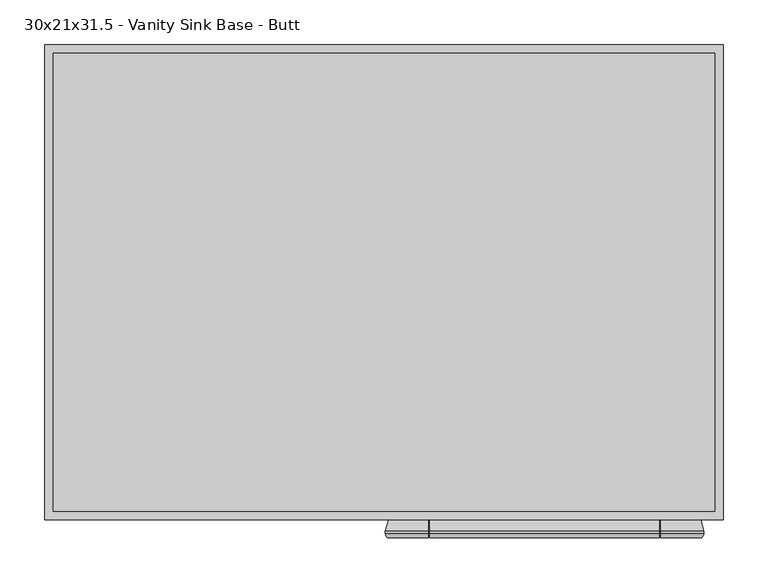
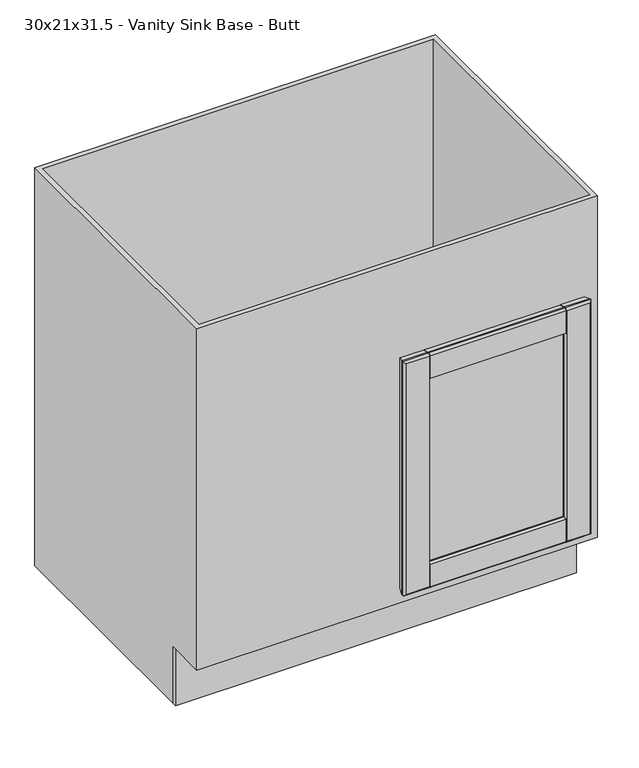
"""IFC4 building model written with IfcOpenShell, lengths in millimetres: furniture geometry, Cabinet-Base-Merillat-Double_Door-Marlin : 30x21x31.5 - Vanity Sink Base - Butt."""

from ifc_helpers import new_model, si_unit, frame, origin, origin_with_axes, place, context, project, spatial, polyline, circle_curve, ellipse_curve, outline, extrude, faceted_brep, source, transform, mapped, element, save
from ifc_brep_helpers import plane_surface, cylinder_surface, advanced_brep


def furniture_30x21x31_5_vanity_sink_base_butt_bc92859f(model_context):
    return source(origin(), model_context, "Body", "SolidModel", [
        advanced_brep(
        [(377.5127049, -625.4496, 609.6), (374.4162124, -629.92, 606.5035075), (374.4162124, -629.92, 142.7964925), (377.5127049, -625.4496, 139.7), (377.5127049, -622.681, 139.7), (377.5127049, -622.681, 609.6), (374.0075049, -609.6, 143.2052), (374.0075049, -609.6, 606.0948), (329.3115422, -609.6, 561.3988372), (329.3115422, -609.6, 187.9011628), (328.9414105, -610.39375, 188.2712945), (326.8602514, -614.85681, 190.3524535), (326.8602514, -614.85681, 558.9475465), (328.9414105, -610.39375, 561.0287055), (328.2600209, -617.0969093, 188.952684), (328.2600209, -617.0969093, 560.347316), (342.5877049, -617.347, 174.625), (342.5877049, -617.347, 574.675), (342.5877049, -622.173, 174.625), (342.5877049, -622.173, 574.675), (328.2600209, -622.4230907, 188.952684), (328.2600209, -622.4230907, 560.347316), (326.8602514, -624.66319, 190.3524535), (326.8602514, -624.66319, 558.9475465), (328.9414105, -629.12625, 188.2712945), (329.3086747, -629.9138508, 187.9040302), (329.3115422, -629.92, 561.3988372), (328.9414105, -629.12625, 561.0287055), (329.3086747, -629.92, 142.7964925), (329.3086747, -625.4496, 139.7), (23.4216974, -629.92, 142.7964925), (20.3252049, -625.4496, 139.7), (68.4894236, -625.4496, 139.7), (68.4894236, -629.92, 142.7964925), (327.7211747, -625.4496, 139.7), (327.7211747, -629.92, 142.7964925), (70.0769236, -629.92, 142.7964925), (70.0769236, -625.4496, 139.7), (329.3086747, -622.681, 139.7), (20.3252049, -622.681, 139.7), (68.4894236, -622.681, 139.7), (327.7211747, -622.681, 139.7), (70.0769236, -622.681, 139.7), (329.3086747, -609.6, 143.2052), (23.8304049, -609.6, 143.2052), (68.4894236, -609.6, 143.2052), (327.7211747, -609.6, 143.2052), (70.0769236, -609.6, 143.2052), (70.9776584, -614.85681, 190.3524535), (327.7211747, -610.39375, 188.2712945), (327.7211747, -609.6, 187.9011628), (70.0769236, -609.6, 187.9011628), (70.0769236, -610.39375, 188.2712945), (68.8964994, -610.39375, 188.2712945), (69.577889, -617.0969093, 188.952684), (55.2502049, -617.347, 174.625), (55.2502049, -622.173, 174.625), (69.577889, -622.4230907, 188.952684), (70.9776584, -624.66319, 190.3524535), (68.8964994, -629.12625, 188.2712945), (70.0769236, -629.12625, 188.2712945), (70.0769236, -629.92, 187.9011628), (327.7211747, -629.92, 187.9011628), (327.7211747, -629.12625, 188.2712945), (23.4216974, -629.92, 606.5035075), (20.3252049, -625.4496, 609.6), (20.3252049, -622.681, 609.6), (23.8304049, -609.6, 606.0948), (68.5263677, -609.6, 187.9011628), (68.5263677, -609.6, 561.3988372), (68.8964994, -610.39375, 561.0287055), (70.9776584, -614.85681, 558.9475465), (69.577889, -617.0969093, 560.347316), (55.2502049, -617.347, 574.675), (55.2502049, -622.173, 574.675), (69.577889, -622.4230907, 560.347316), (70.9776584, -624.66319, 558.9475465), (68.8964994, -629.12625, 561.0287055), (68.5263677, -629.92, 561.3988372), (68.5263677, -629.92, 187.9011628), (68.4894236, -629.92, 606.5035075), (68.4894236, -625.4496, 609.6), (329.3086747, -625.4496, 609.6), (329.3086747, -629.92, 606.5035075), (70.0769236, -625.4496, 609.6), (70.0769236, -629.92, 606.5035075), (327.7211747, -629.92, 606.5035075), (327.7211747, -625.4496, 609.6), (68.4894236, -622.681, 609.6), (329.3086747, -622.681, 609.6), (70.0769236, -622.681, 609.6), (327.7211747, -622.681, 609.6), (68.4894236, -609.6, 606.0948), (329.3086747, -609.6, 606.0948), (70.0769236, -609.6, 606.0948), (327.7211747, -609.6, 606.0948), (70.0769236, -609.6, 561.3988372), (327.7211747, -609.6, 561.3988372), (70.0769236, -610.39375, 561.0287055), (327.7211747, -610.39375, 561.0287055), (327.7211747, -629.12625, 561.0287055), (327.7211747, -629.92, 561.3988372), (70.0769236, -629.92, 561.3988372), (70.0769236, -629.12625, 561.0287055), (70.0769236, -610.39375, 605.4857412), (70.0769236, -622.7855037, 608.80625), (70.0769236, -625.4496, 608.80625), (70.0769236, -629.12625, 606.3526052), (68.4894236, -629.12625, 561.0287055), (68.4894236, -629.12625, 606.3526052), (68.4894236, -625.4496, 608.80625), (68.4894236, -622.7855037, 608.80625), (68.4894236, -610.39375, 605.4857412), (68.4894236, -610.39375, 561.0287055), (329.3086747, -610.39375, 561.0287055), (329.3086747, -610.39375, 605.4857412), (329.3086747, -622.7855037, 608.80625), (329.3086747, -625.4496, 608.80625), (329.3086747, -629.12625, 606.3526052), (329.3086747, -629.12625, 561.0287055), (327.7211747, -629.12625, 606.3526052), (327.7211747, -625.4496, 608.80625), (327.7211747, -622.7855037, 608.80625), (327.7211747, -610.39375, 605.4857412), (329.3086747, -629.12625, 188.2712945), (329.3086747, -629.12625, 142.9473948), (329.3086747, -625.4496, 140.49375), (329.3086747, -622.7855037, 140.49375), (329.3086747, -610.39375, 143.8142588), (329.3086747, -610.39375, 188.2712945), (327.7211747, -610.39375, 143.8142588), (327.7211747, -622.7855037, 140.49375), (327.7211747, -625.4496, 140.49375), (327.7211747, -629.12625, 142.9473948), (70.0769236, -629.12625, 142.9473948), (70.0769236, -625.4496, 140.49375), (70.0769236, -622.7855037, 140.49375), (70.0769236, -610.39375, 143.8142588), (68.4894236, -629.12625, 188.2712945), (68.4894236, -610.39375, 188.2712945), (68.4894236, -610.39375, 143.8142588), (68.4894236, -622.7855037, 140.49375), (68.4894236, -625.4496, 140.49375), (68.4894236, -629.12625, 142.9473948)],
        [
            (0, 1, ellipse_curve(frame((372.7375049, -625.4496, 604.8248), z_axis=(0.7071067811865475, 0.0, -0.7071067811865475), x_axis=(0.7071067811865474, 0.0, 0.7071067811865476)), 6.7531526, 4.7752)),
            (1, 2),
            (2, 3, ellipse_curve(frame((372.7375049, -625.4496, 144.4752), z_axis=(0.7071067811865475, 0.0, 0.7071067811865475), x_axis=(-0.7071067811865474, 0.0, 0.7071067811865476)), 6.7531526, 4.7752)),
            (3, 0),
            (3, 4),
            (4, 5),
            (5, 0),
            (4, 6),
            (6, 7),
            (7, 5),
            (8, 9),
            (9, 10),
            (10, 11),
            (11, 12),
            (12, 13),
            (13, 8),
            (11, 14, ellipse_curve(frame((328.2875049, -615.5223492, 188.9252), z_axis=(0.7071067811865475, 0.0, 0.7071067811865475), x_axis=(-0.7071067811865474, 0.0, 0.7071067811865476)), 2.2271035, 1.5748)),
            (14, 15),
            (15, 12, ellipse_curve(frame((328.2875049, -615.5223492, 560.3748), z_axis=(0.7071067811865475, 0.0, -0.7071067811865475), x_axis=(0.7071067811865474, 0.0, 0.7071067811865476)), 2.2271035, 1.5748)),
            (14, 16),
            (16, 17),
            (17, 15),
            (16, 18),
            (18, 19),
            (19, 17),
            (18, 20),
            (20, 21),
            (21, 19),
            (20, 22, ellipse_curve(frame((328.2875049, -623.9976508, 188.9252), z_axis=(0.7071067811865475, 0.0, 0.7071067811865475), x_axis=(-0.7071067811865474, 0.0, 0.7071067811865476)), 2.2271035, 1.5748)),
            (22, 23),
            (23, 21, ellipse_curve(frame((328.2875049, -623.9976508, 560.3748), z_axis=(0.7071067811865475, 0.0, -0.7071067811865475), x_axis=(0.7071067811865474, 0.0, 0.7071067811865476)), 2.2271035, 1.5748)),
            (22, 24),
            (24, 25),
            (25, 26),
            (26, 27),
            (27, 23),
            (2, 28),
            (28, 29, circle_curve(frame((329.3086747, -625.4496, 144.4752), z_axis=(1.0, 0.0, 0.0), x_axis=(0.0, 1.0, 0.0)), 4.7752)),
            (29, 3),
            (30, 31, ellipse_curve(frame((25.1004049, -625.4496, 144.4752), z_axis=(0.7071067811865475, 0.0, -0.7071067811865475), x_axis=(0.7071067811865476, 0.0, 0.7071067811865474)), 6.7531526, 4.7752)),
            (31, 32),
            (32, 33, circle_curve(frame((68.4894236, -625.4496, 144.4752), z_axis=(-1.0, 0.0, 0.0), x_axis=(0.0, 1.0, 0.0)), 4.7752)),
            (33, 30),
            (34, 35, circle_curve(frame((327.7211747, -625.4496, 144.4752), z_axis=(-1.0, 0.0, 0.0), x_axis=(0.0, 1.0, 0.0)), 4.7752)),
            (35, 36),
            (36, 37, circle_curve(frame((70.0769236, -625.4496, 144.4752), z_axis=(1.0, 0.0, 0.0), x_axis=(0.0, 1.0, 0.0)), 4.7752)),
            (37, 34),
            (29, 38),
            (38, 4),
            (31, 39),
            (39, 40),
            (40, 32),
            (41, 34),
            (37, 42),
            (42, 41),
            (38, 43),
            (43, 6),
            (39, 44),
            (44, 45),
            (45, 40),
            (46, 41),
            (42, 47),
            (47, 46),
            (48, 11),
            (10, 49),
            (49, 50),
            (50, 51),
            (51, 52),
            (52, 53),
            (53, 48),
            (48, 54, ellipse_curve(frame((69.5504049, -615.5223492, 188.9252), z_axis=(0.7071067811865475, 0.0, -0.7071067811865475), x_axis=(0.7071067811865476, 0.0, 0.7071067811865474)), 2.2271035, 1.5748)),
            (54, 14),
            (54, 55),
            (55, 16),
            (55, 56),
            (56, 18),
            (56, 57),
            (57, 20),
            (57, 58, ellipse_curve(frame((69.5504049, -623.9976508, 188.9252), z_axis=(0.7071067811865475, 0.0, -0.7071067811865475), x_axis=(0.7071067811865476, 0.0, 0.7071067811865474)), 2.2271035, 1.5748)),
            (58, 22),
            (58, 59),
            (59, 60),
            (60, 61),
            (61, 62),
            (62, 63),
            (63, 24),
            (30, 64),
            (64, 65, ellipse_curve(frame((25.1004049, -625.4496, 604.8248), z_axis=(-0.7071067811865475, 0.0, -0.7071067811865475), x_axis=(0.7071067811865474, 0.0, -0.7071067811865476)), 6.7531526, 4.7752)),
            (65, 31),
            (65, 66),
            (66, 39),
            (66, 67),
            (67, 44),
            (68, 69),
            (69, 70),
            (70, 71),
            (71, 48),
            (53, 68),
            (71, 72, ellipse_curve(frame((69.5504049, -615.5223492, 560.3748), z_axis=(-0.7071067811865475, 0.0, -0.7071067811865475), x_axis=(0.7071067811865474, 0.0, -0.7071067811865476)), 2.2271035, 1.5748)),
            (72, 54),
            (72, 73),
            (73, 55),
            (73, 74),
            (74, 56),
            (74, 75),
            (75, 57),
            (75, 76, ellipse_curve(frame((69.5504049, -623.9976508, 560.3748), z_axis=(-0.7071067811865475, 0.0, -0.7071067811865475), x_axis=(0.7071067811865474, 0.0, -0.7071067811865476)), 2.2271035, 1.5748)),
            (76, 58),
            (76, 77),
            (77, 78),
            (78, 79),
            (79, 59),
            (64, 80),
            (80, 81, circle_curve(frame((68.4894236, -625.4496, 604.8248), z_axis=(-1.0, 0.0, 0.0), x_axis=(0.0, 1.0, 0.0)), 4.7752)),
            (81, 65),
            (0, 82),
            (82, 83, circle_curve(frame((329.3086747, -625.4496, 604.8248), z_axis=(1.0, 0.0, 0.0), x_axis=(0.0, 1.0, 0.0)), 4.7752)),
            (83, 1),
            (84, 85, circle_curve(frame((70.0769236, -625.4496, 604.8248), z_axis=(1.0, 0.0, 0.0), x_axis=(0.0, 1.0, 0.0)), 4.7752)),
            (85, 86),
            (86, 87, circle_curve(frame((327.7211747, -625.4496, 604.8248), z_axis=(-1.0, 0.0, 0.0), x_axis=(0.0, 1.0, 0.0)), 4.7752)),
            (87, 84),
            (81, 88),
            (88, 66),
            (5, 89),
            (89, 82),
            (90, 84),
            (87, 91),
            (91, 90),
            (88, 92),
            (92, 67),
            (7, 93),
            (93, 89),
            (94, 90),
            (91, 95),
            (95, 94),
            (43, 9),
            (8, 93),
            (92, 69),
            (68, 45),
            (96, 94),
            (95, 97),
            (97, 96),
            (50, 46),
            (47, 51),
            (12, 71),
            (70, 98),
            (98, 96),
            (97, 99),
            (99, 13),
            (15, 72),
            (17, 73),
            (19, 74),
            (21, 75),
            (23, 76),
            (27, 100),
            (100, 101),
            (101, 102),
            (102, 103),
            (103, 77),
            (83, 26),
            (25, 28),
            (33, 79),
            (78, 80),
            (85, 102),
            (101, 86),
            (35, 62),
            (61, 36),
            (98, 104),
            (104, 105),
            (105, 106),
            (106, 107, circle_curve(frame((70.0769236, -625.4496, 604.8248), z_axis=(1.0, 0.0, 0.0), x_axis=(0.0, 0.0, 1.0)), 3.98145)),
            (107, 103),
            (78, 108),
            (108, 109),
            (109, 110, circle_curve(frame((68.4894236, -625.4496, 604.8248), z_axis=(-1.0, 0.0, 0.0), x_axis=(0.0, 0.0, 1.0)), 3.98145)),
            (110, 111),
            (111, 112),
            (112, 113),
            (113, 69),
            (77, 108),
            (107, 109),
            (106, 110),
            (105, 111),
            (104, 112),
            (70, 113),
            (8, 114),
            (114, 115),
            (115, 116),
            (116, 117),
            (117, 118, circle_curve(frame((329.3086747, -625.4496, 604.8248), z_axis=(1.0, 0.0, 0.0), x_axis=(0.0, 0.0, 1.0)), 3.98145)),
            (118, 119),
            (119, 26),
            (100, 120),
            (120, 121, circle_curve(frame((327.7211747, -625.4496, 604.8248), z_axis=(-1.0, 0.0, 0.0), x_axis=(0.0, 0.0, 1.0)), 3.98145)),
            (121, 122),
            (122, 123),
            (123, 99),
            (119, 27),
            (118, 120),
            (117, 121),
            (116, 122),
            (115, 123),
            (114, 13),
            (25, 124),
            (124, 125),
            (125, 126, circle_curve(frame((329.3086747, -625.4496, 144.4752), z_axis=(1.0, 0.0, 0.0), x_axis=(0.0, 0.0, 1.0)), 3.98145)),
            (126, 127),
            (127, 128),
            (128, 129),
            (129, 9),
            (49, 130),
            (130, 131),
            (131, 132),
            (132, 133, circle_curve(frame((327.7211747, -625.4496, 144.4752), z_axis=(-1.0, 0.0, 0.0), x_axis=(0.0, 0.0, 1.0)), 3.98145)),
            (133, 63),
            (129, 10),
            (128, 130),
            (127, 131),
            (126, 132),
            (125, 133),
            (124, 24),
            (60, 134),
            (134, 135, circle_curve(frame((70.0769236, -625.4496, 144.4752), z_axis=(1.0, 0.0, 0.0), x_axis=(0.0, 0.0, 1.0)), 3.98145)),
            (135, 136),
            (136, 137),
            (137, 52),
            (138, 79),
            (68, 139),
            (139, 140),
            (140, 141),
            (141, 142),
            (142, 143, circle_curve(frame((68.4894236, -625.4496, 144.4752), z_axis=(-1.0, 0.0, 0.0), x_axis=(0.0, 0.0, 1.0)), 3.98145)),
            (143, 138),
            (138, 59),
            (53, 139),
            (137, 140),
            (136, 141),
            (135, 142),
            (134, 143),
        ],
        [
            cylinder_surface(frame((372.7375049, -625.4496, 609.6), z_axis=(0.0, 0.0, 1.0), x_axis=(0.0, 1.0, 0.0)), 4.7752),
            plane_surface(frame((377.5127049, -625.4496, 609.6), z_axis=(1.0, 0.0, 0.0), x_axis=(0.0, 0.0, -1.0))),
            plane_surface(frame((377.5127049, -622.681, 609.6), z_axis=(0.9659229350723619, 0.25882983502910506, 0.0), x_axis=(0.0, 0.0, -1.0))),
            plane_surface(frame((329.3115422, -609.6, 561.3988372), z_axis=(-0.9063077870366099, 0.4226182617407856, 0.0), x_axis=(0.0, 0.0, -1.0))),
            cylinder_surface(frame((328.2875049, -615.5223492, 609.6), z_axis=(0.0, 0.0, 1.0000000000000002), x_axis=(-0.01745240643729364, -0.9998476951563912, 0.0)), 1.5748),
            plane_surface(frame((328.2600209, -617.0969093, 560.347316), z_axis=(-0.017452406437322144, -0.9998476951563906, 0.0), x_axis=(0.0, 0.0, -1.0))),
            plane_surface(frame((342.5877049, -617.347, 574.675), z_axis=(-1.0, 0.0, 0.0), x_axis=(0.0, 0.0, -1.0))),
            plane_surface(frame((342.5877049, -622.173, 574.675), z_axis=(-0.01745240643727848, 0.9998476951563914, 0.0), x_axis=(0.0, 0.0, -1.0))),
            cylinder_surface(frame((328.2875049, -623.9976508, 609.6), z_axis=(0.0, 0.0, 1.0000000000000002), x_axis=(-0.9063077870367326, -0.42261826174052236, 0.0)), 1.5748),
            plane_surface(frame((326.8602514, -624.66319, 558.9475465), z_axis=(-0.9063077870366333, -0.4226182617407352, 0.0), x_axis=(0.0, 0.0, -1.0))),
            cylinder_surface(frame((377.5127049, -625.4496, 144.4752), z_axis=(1.0, 0.0, 0.0), x_axis=(0.0, 1.0, 0.0)), 4.7752),
            plane_surface(frame((377.5127049, -625.4496, 139.7), z_axis=(0.0, 0.0, -1.0), x_axis=(-1.0, 0.0, 0.0))),
            plane_surface(frame((377.5127049, -622.681, 139.7), z_axis=(0.0, 0.25882983502910506, -0.9659229350723619), x_axis=(-1.0, 0.0, 0.0))),
            plane_surface(frame((329.3115422, -609.6, 187.9011628), z_axis=(0.0, 0.4226182617407856, 0.9063077870366099), x_axis=(-1.0, 0.0, 0.0))),
            cylinder_surface(frame((377.5127049, -615.5223492, 188.9252), z_axis=(1.0000000000000002, 0.0, 0.0), x_axis=(0.0, -0.9998476951563912, 0.01745240643729364)), 1.5748),
            plane_surface(frame((328.2600209, -617.0969093, 188.952684), z_axis=(0.0, -0.9998476951563906, 0.017452406437322144), x_axis=(-1.0, 0.0, 0.0))),
            plane_surface(frame((342.5877049, -617.347, 174.625), z_axis=(0.0, 0.0, 1.0), x_axis=(-1.0, 0.0, 0.0))),
            plane_surface(frame((342.5877049, -622.173, 174.625), z_axis=(0.0, 0.9998476951563914, 0.01745240643727848), x_axis=(-1.0, 0.0, 0.0))),
            cylinder_surface(frame((377.5127049, -623.9976508, 188.9252), z_axis=(1.0000000000000002, 0.0, 0.0), x_axis=(0.0, -0.42261826174052236, 0.9063077870367326)), 1.5748),
            plane_surface(frame((326.8602514, -624.66319, 190.3524535), z_axis=(0.0, -0.4226182617407352, 0.9063077870366333), x_axis=(-1.0, 0.0, 0.0))),
            cylinder_surface(frame((25.1004049, -625.4496, 139.7), z_axis=(0.0, 0.0, -1.0), x_axis=(0.0, 1.0, 0.0)), 4.7752),
            plane_surface(frame((20.3252049, -625.4496, 139.7), z_axis=(-1.0, 0.0, 0.0), x_axis=(0.0, 0.0, 1.0))),
            plane_surface(frame((20.3252049, -622.681, 139.7), z_axis=(-0.9659229350723619, 0.25882983502910506, 0.0), x_axis=(0.0, 0.0, 1.0))),
            plane_surface(frame((68.5263677, -609.6, 187.9011628), z_axis=(0.9063077870366099, 0.4226182617407856, 0.0), x_axis=(0.0, 0.0, 1.0))),
            cylinder_surface(frame((69.5504049, -615.5223492, 139.7), z_axis=(0.0, 0.0, -1.0000000000000002), x_axis=(0.01745240643729364, -0.9998476951563912, 0.0)), 1.5748),
            plane_surface(frame((69.577889, -617.0969093, 188.952684), z_axis=(0.017452406437322144, -0.9998476951563906, 0.0), x_axis=(0.0, 0.0, 1.0))),
            plane_surface(frame((55.2502049, -617.347, 174.625), z_axis=(1.0, 0.0, 0.0), x_axis=(0.0, 0.0, 1.0))),
            plane_surface(frame((55.2502049, -622.173, 174.625), z_axis=(0.01745240643727848, 0.9998476951563914, 0.0), x_axis=(0.0, 0.0, 1.0))),
            cylinder_surface(frame((69.5504049, -623.9976508, 139.7), z_axis=(0.0, 0.0, -1.0000000000000002), x_axis=(0.9063077870367326, -0.42261826174052236, 0.0)), 1.5748),
            plane_surface(frame((70.9776584, -624.66319, 190.3524535), z_axis=(0.9063077870366333, -0.4226182617407352, 0.0), x_axis=(0.0, 0.0, 1.0))),
            cylinder_surface(frame((20.3252049, -625.4496, 604.8248), z_axis=(-1.0, 0.0, 0.0), x_axis=(0.0, 1.0, 0.0)), 4.7752),
            plane_surface(frame((20.3252049, -625.4496, 609.6), z_axis=(0.0, 0.0, 1.0), x_axis=(1.0, 0.0, 0.0))),
            plane_surface(frame((20.3252049, -622.681, 609.6), z_axis=(0.0, 0.25882983502910506, 0.9659229350723619), x_axis=(1.0, 0.0, 0.0))),
            plane_surface(frame((23.8304049, -609.6, 606.0948), z_axis=(0.0, 1.0, 0.0), x_axis=(1.0, 0.0, 0.0))),
            plane_surface(frame((68.5263677, -609.6, 561.3988372), z_axis=(0.0, 0.4226182617407856, -0.9063077870366099), x_axis=(1.0, 0.0, 0.0))),
            cylinder_surface(frame((20.3252049, -615.5223492, 560.3748), z_axis=(-1.0000000000000002, 0.0, 0.0), x_axis=(0.0, -0.9998476951563912, -0.01745240643729364)), 1.5748),
            plane_surface(frame((69.577889, -617.0969093, 560.347316), z_axis=(0.0, -0.9998476951563906, -0.017452406437322144), x_axis=(1.0, 0.0, 0.0))),
            plane_surface(frame((55.2502049, -617.347, 574.675), z_axis=(0.0, 0.0, -1.0), x_axis=(1.0, 0.0, 0.0))),
            plane_surface(frame((55.2502049, -622.173, 574.675), z_axis=(0.0, 0.9998476951563914, -0.01745240643727848), x_axis=(1.0, 0.0, 0.0))),
            cylinder_surface(frame((20.3252049, -623.9976508, 560.3748), z_axis=(-1.0000000000000002, 0.0, 0.0), x_axis=(0.0, -0.42261826174052236, -0.9063077870367326)), 1.5748),
            plane_surface(frame((70.9776584, -624.66319, 558.9475465), z_axis=(0.0, -0.4226182617407352, -0.9063077870366333), x_axis=(1.0, 0.0, 0.0))),
            plane_surface(frame((68.5263677, -629.92, 561.3988372), z_axis=(0.0, -1.0, 0.0), x_axis=(1.0, 0.0, 0.0))),
            plane_surface(frame((70.0769236, -629.92, 561.3988372), z_axis=(-1.0, 0.0, 0.0), x_axis=(0.0, 0.9063077870366297, -0.42261826174074285))),
            plane_surface(frame((68.4894236, -629.92, 561.3988372), z_axis=(1.0, 0.0, 0.0), x_axis=(0.0, -0.9063077870366297, 0.42261826174074285))),
            plane_surface(frame((70.0769236, -629.92, 561.3988372), z_axis=(0.0, 0.42261826174074285, 0.9063077870366297), x_axis=(-1.0, 0.0, 0.0))),
            plane_surface(frame((70.0769236, -629.12625, 561.0287055), z_axis=(0.0, -1.0, 0.0), x_axis=(-1.0, 0.0, 0.0))),
            cylinder_surface(frame((68.4894236, -625.4496, 604.8248), z_axis=(-1.0, 0.0, 0.0), x_axis=(0.0, 0.0, 1.0)), 3.98145),
            plane_surface(frame((70.0769236, -625.4496, 608.80625), z_axis=(0.0, 0.0, 1.0), x_axis=(-1.0, 0.0, 0.0))),
            plane_surface(frame((70.0769236, -622.7855037, 608.80625), z_axis=(0.0, 0.25882983502916584, 0.9659229350723456), x_axis=(-1.0, 0.0, 0.0))),
            plane_surface(frame((70.0769236, -610.39375, 605.4857412), z_axis=(0.0, 1.0, 0.0), x_axis=(-1.0, 0.0, 0.0))),
            plane_surface(frame((70.0769236, -610.39375, 561.0287055), z_axis=(0.0, -0.42261826174077916, 0.9063077870366127), x_axis=(-1.0, 0.0, 0.0))),
            plane_surface(frame((329.3086747, -629.92, 561.3988372), z_axis=(-1.0, 0.0, 0.0), x_axis=(0.0, 0.9063077870366253, -0.4226182617407524))),
            plane_surface(frame((327.7211747, -629.92, 561.3988372), z_axis=(1.0, 0.0, 0.0), x_axis=(0.0, -0.9063077870366253, 0.4226182617407524))),
            plane_surface(frame((329.3086747, -629.92, 561.3988372), z_axis=(0.0, 0.4226182617407524, 0.9063077870366253), x_axis=(-1.0, 0.0, 0.0))),
            plane_surface(frame((329.3086747, -629.12625, 561.0287055), z_axis=(0.0, -1.0, 0.0), x_axis=(-1.0, 0.0, 0.0))),
            cylinder_surface(frame((327.7211747, -625.4496, 604.8248), z_axis=(-1.0, 0.0, 0.0), x_axis=(0.0, 0.0, 1.0)), 3.98145),
            plane_surface(frame((329.3086747, -625.4496, 608.80625), z_axis=(0.0, 0.0, 1.0), x_axis=(-1.0, 0.0, 0.0))),
            plane_surface(frame((329.3086747, -622.7855037, 608.80625), z_axis=(0.0, 0.25882983502916573, 0.9659229350723457), x_axis=(-1.0, 0.0, 0.0))),
            plane_surface(frame((329.3086747, -610.39375, 605.4857412), z_axis=(0.0, 1.0, 0.0), x_axis=(-1.0, 0.0, 0.0))),
            plane_surface(frame((329.3086747, -610.39375, 561.0287055), z_axis=(0.0, -0.4226182617407701, 0.906307787036617), x_axis=(-1.0, 0.0, 0.0))),
            plane_surface(frame((329.3086747, -625.4496, 149.2504), z_axis=(-1.0, 0.0, 0.0), x_axis=(0.0, -1.0, 0.0))),
            plane_surface(frame((327.7211747, -625.4496, 149.2504), z_axis=(1.0, 0.0, 0.0), x_axis=(0.0, 1.0, 0.0))),
            plane_surface(frame((329.3086747, -609.6, 187.9011628), z_axis=(0.0, -0.4226182617407918, -0.906307787036607), x_axis=(-1.0, 0.0, 0.0))),
            plane_surface(frame((329.3086747, -610.39375, 188.2712945), z_axis=(0.0, 1.0, 0.0), x_axis=(-1.0, 0.0, 0.0))),
            plane_surface(frame((329.3086747, -610.39375, 143.8142588), z_axis=(0.0, 0.25882983502943896, -0.9659229350722724), x_axis=(-1.0, 0.0, 0.0))),
            plane_surface(frame((329.3086747, -622.7855037, 140.49375), z_axis=(0.0, 0.0, -1.0), x_axis=(-1.0, 0.0, 0.0))),
            cylinder_surface(frame((327.7211747, -625.4496, 144.4752), z_axis=(-1.0, 0.0, 0.0), x_axis=(0.0, 0.0, 1.0)), 3.98145),
            plane_surface(frame((329.3086747, -629.12625, 142.9473948), z_axis=(0.0, -1.0, 0.0), x_axis=(-1.0, 0.0, 0.0))),
            plane_surface(frame((329.3086747, -629.12625, 188.2712945), z_axis=(0.0, 0.42261826174073464, -0.9063077870366336), x_axis=(-1.0, 0.0, 0.0))),
            plane_surface(frame((70.0769236, -629.12625, 188.2712945), z_axis=(-1.0, 0.0, 0.0), x_axis=(0.0, -0.9063077870366323, -0.4226182617407374))),
            plane_surface(frame((68.4894236, -629.12625, 188.2712945), z_axis=(1.0, 0.0, 0.0), x_axis=(0.0, 0.9063077870366323, 0.4226182617407374))),
            plane_surface(frame((70.0769236, -629.12625, 188.2712945), z_axis=(0.0, 0.4226182617407374, -0.9063077870366323), x_axis=(-1.0, 0.0, 0.0))),
            plane_surface(frame((70.0769236, -609.6, 187.9011628), z_axis=(0.0, -0.42261826174081374, -0.9063077870365968), x_axis=(-1.0, 0.0, 0.0))),
            plane_surface(frame((70.0769236, -610.39375, 188.2712945), z_axis=(0.0, 1.0, 0.0), x_axis=(-1.0, 0.0, 0.0))),
            plane_surface(frame((70.0769236, -610.39375, 143.8142588), z_axis=(0.0, 0.25882983502943885, -0.9659229350722726), x_axis=(-1.0, 0.0, 0.0))),
            plane_surface(frame((70.0769236, -622.7855037, 140.49375), z_axis=(0.0, 0.0, -1.0), x_axis=(-1.0, 0.0, 0.0))),
            cylinder_surface(frame((68.4894236, -625.4496, 144.4752), z_axis=(-1.0, 0.0, 0.0), x_axis=(0.0, 0.0, 1.0)), 3.98145),
            plane_surface(frame((70.0769236, -629.12625, 142.9473948), z_axis=(0.0, -1.0, 0.0), x_axis=(-1.0, 0.0, 0.0))),
        ],
        [
            (0, [[1, 2, 3, 4]]),
            (1, [[-4, 5, 6, 7]]),
            (2, [[-6, 8, 9, 10]]),
            (3, [[11, 12, 13, 14, 15, 16]]),
            (4, [[-14, 17, 18, 19]]),
            (5, [[-18, 20, 21, 22]]),
            (6, [[-21, 23, 24, 25]]),
            (7, [[-24, 26, 27, 28]]),
            (8, [[-27, 29, 30, 31]]),
            (9, [[-30, 32, 33, 34, 35, 36]]),
            (10, [[-3, 37, 38, 39]]),
            (10, [[40, 41, 42, 43]]),
            (10, [[44, 45, 46, 47]]),
            (11, [[-5, -39, 48, 49]]),
            (11, [[50, 51, 52, -41]]),
            (11, [[53, -47, 54, 55]]),
            (12, [[-8, -49, 56, 57]]),
            (12, [[58, 59, 60, -51]]),
            (12, [[61, -55, 62, 63]]),
            (13, [[64, -13, 65, 66, 67, 68, 69, 70]]),
            (14, [[-17, -64, 71, 72]]),
            (15, [[-20, -72, 73, 74]]),
            (16, [[-23, -74, 75, 76]]),
            (17, [[-26, -76, 77, 78]]),
            (18, [[-29, -78, 79, 80]]),
            (19, [[-80, 81, 82, 83, 84, 85, 86, -32]]),
            (20, [[-40, 87, 88, 89]]),
            (21, [[-50, -89, 90, 91]]),
            (22, [[-58, -91, 92, 93]]),
            (23, [[94, 95, 96, 97, -70, 98]]),
            (24, [[-71, -97, 99, 100]]),
            (25, [[-73, -100, 101, 102]]),
            (26, [[-75, -102, 103, 104]]),
            (27, [[-77, -104, 105, 106]]),
            (28, [[-79, -106, 107, 108]]),
            (29, [[-108, 109, 110, 111, 112, -81]]),
            (30, [[-88, 113, 114, 115]]),
            (30, [[-1, 116, 117, 118]]),
            (30, [[119, 120, 121, 122]]),
            (31, [[-90, -115, 123, 124]]),
            (31, [[-7, 125, 126, -116]]),
            (31, [[127, -122, 128, 129]]),
            (32, [[-92, -124, 130, 131]]),
            (32, [[-10, 132, 133, -125]]),
            (32, [[134, -129, 135, 136]]),
            (33, [[-9, -57, 137, -11, 138, -132]]),
            (33, [[-93, -131, 139, -94, 140, -59]]),
            (33, [[141, -136, 142, 143]]),
            (33, [[144, -63, 145, -67]]),
            (34, [[146, -96, 147, 148, -143, 149, 150, -15]]),
            (35, [[-19, 151, -99, -146]]),
            (36, [[-22, 152, -101, -151]]),
            (37, [[-25, 153, -103, -152]]),
            (38, [[-28, 154, -105, -153]]),
            (39, [[-31, 155, -107, -154]]),
            (40, [[-155, -36, 156, 157, 158, 159, 160, -109]]),
            (41, [[-2, -118, 161, -34, 162, -37]]),
            (41, [[-87, -43, 163, -111, 164, -113]]),
            (41, [[165, -158, 166, -120]]),
            (41, [[167, -84, 168, -45]]),
            (42, [[169, 170, 171, 172, 173, -159, -165, -119, -127, -134, -141, -148]]),
            (43, [[174, 175, 176, 177, 178, 179, 180, -139, -130, -123, -114, -164]]),
            (44, [[-174, -110, 181]]),
            (45, [[-173, 182, -175, -181, -160]]),
            (46, [[-172, 183, -176, -182]]),
            (47, [[-171, 184, -177, -183]]),
            (48, [[-170, 185, -178, -184]]),
            (49, [[-169, -147, 186, -179, -185]]),
            (50, [[-180, -186, -95]]),
            (51, [[187, 188, 189, 190, 191, 192, 193, -161, -117, -126, -133, -138]]),
            (52, [[194, 195, 196, 197, 198, -149, -142, -135, -128, -121, -166, -157]]),
            (53, [[-193, 199, -35]]),
            (54, [[-192, 200, -194, -156, -199]]),
            (55, [[-191, 201, -195, -200]]),
            (56, [[-190, 202, -196, -201]]),
            (57, [[-189, 203, -197, -202]]),
            (58, [[-188, 204, -150, -198, -203]]),
            (59, [[-187, -16, -204]]),
            (60, [[205, 206, 207, 208, 209, 210, 211, -137, -56, -48, -38, -162]]),
            (61, [[212, 213, 214, 215, 216, -85, -167, -44, -53, -61, -144, -66]]),
            (62, [[-211, 217, -12]]),
            (63, [[-210, 218, -212, -65, -217]]),
            (64, [[-209, 219, -213, -218]]),
            (65, [[-208, 220, -214, -219]]),
            (66, [[-207, 221, -215, -220]]),
            (67, [[-206, 222, -86, -216, -221]]),
            (68, [[-205, -33, -222]]),
            (69, [[223, 224, 225, 226, 227, -68, -145, -62, -54, -46, -168, -83]]),
            (70, [[228, -163, -42, -52, -60, -140, 229, 230, 231, 232, 233, 234]]),
            (71, [[-228, 235, -112]]),
            (72, [[-229, -98, 236]]),
            (73, [[-227, 237, -230, -236, -69]]),
            (74, [[-226, 238, -231, -237]]),
            (75, [[-225, 239, -232, -238]]),
            (76, [[-224, 240, -233, -239]]),
            (77, [[-223, -82, -235, -234, -240]]),
        ],
    ),
        extrude(outline(polyline([(55.2502049, -622.173), (55.2502049, -617.347), (342.5877049, -617.347), (342.5877049, -622.173), (55.2502049, -622.173)])), frame((0.0, 0.0, 174.625), z_axis=(0.0, 0.0, 1.0), x_axis=(1.0, 0.0, 0.0)), (0.0, 0.0, 1.0), 400.05),
        faceted_brep([(399.7377049, -76.2, 0.0), (399.7377049, -529.43125, 0.0), (390.2127049, -529.43125, 0.0), (390.2127049, -85.725, 0.0), (-352.7372951, -85.725, 0.0), (-352.7372951, -529.43125, 0.0), (-362.2622951, -529.43125, 0.0), (-362.2622951, -76.2, 0.0), (-362.2622951, -76.2, 800.1), (399.7377049, -76.2, 800.1), (-362.2622951, -529.43125, 114.3), (-362.2622951, -609.6, 114.3), (-362.2622951, -609.6, 800.1), (399.7377049, -609.6, 800.1), (399.7377049, -609.6, 114.3), (399.7377049, -529.43125, 114.3), (390.2127049, -529.43125, 114.3), (390.2127049, -85.725, 114.3), (390.2127049, -600.075, 800.1), (390.2127049, -85.725, 800.1), (390.2127049, -85.725, 123.825), (390.2127049, -600.075, 123.825), (-352.7372951, -85.725, 114.3), (-352.7372951, -529.43125, 114.3), (-352.7372951, -85.725, 800.1), (-352.7372951, -600.075, 800.1), (-352.7372951, -600.075, 123.825), (-352.7372951, -85.725, 123.825)], [[[0, 1, 2, 3, 4, 5, 6, 7]], [[0, 7, 8, 9]], [[7, 6, 10, 11, 12, 8]], [[1, 0, 9, 13, 14, 15]], [[3, 2, 16, 17]], [[18, 19, 20, 21]], [[5, 4, 22, 23]], [[24, 25, 26, 27]], [[4, 3, 17, 22]], [[19, 24, 27, 20]], [[9, 8, 12, 13], [19, 18, 25, 24]], [[14, 11, 10, 23, 22, 17, 16, 15]], [[13, 12, 11, 14]], [[25, 18, 21, 26]], [[6, 5, 23, 10]], [[2, 1, 15, 16]], [[21, 20, 27, 26]]]),
        extrude(outline(polyline([(399.7377049, -529.43125), (399.7377049, -538.95625), (-362.2622951, -538.95625), (-362.2622951, -529.43125), (399.7377049, -529.43125)])), origin_with_axes(), (0.0, 0.0, 1.0), 114.3),
    ])


if __name__ == "__main__":
    model = new_model("IFC4")
    model_context = context("Model", 3, world=origin())
    ifc_project = project(units=[si_unit("LENGTHUNIT", "METRE", prefix="MILLI")], contexts=[model_context])
    site = spatial("IfcSite", under=ifc_project)
    building = spatial("IfcBuilding", under=site)
    placement = place(None, origin())
    furniture_30x21x31_5_vanity_sink_base_butt_shape = furniture_30x21x31_5_vanity_sink_base_butt_bc92859f(model_context)
    element("IfcFurniture", 1, ObjectType="Cabinet-Base-Merillat-Double_Door-Marlin : 30x21x31.5 - Vanity Sink Base - Butt", at=placement, inside=building, context=model_context, shape_type="MappedRepresentation", body=[
        mapped(furniture_30x21x31_5_vanity_sink_base_butt_shape, transform((0.0, 0.0, 0.0), x_axis=(1.0, 0.0, 0.0), y_axis=(0.0, 1.0, 0.0), z_axis=(0.0, 0.0, 1.0))),
    ])
    save(model, "model.ifc")

# Revit data of these elements
# Type "Cabinet-Base-Merillat-Double_Door-Marlin : 30x21x31.5 - Vanity Sink Base - Butt"
#   URL = "http://www.merillat.com"
#   Toe Kick Note = "Toe Kick Covering is not included. To be purchased Separately."
#   Product Line = "Express"
#   Product Page URL = "http://www.merillat.com//our-products/rooms/bathroom"
#   Product Group = "Vanity Cabinet"
#   Product Documentation Link = "http://merillatbusiness.com/customer-resources/product-line-resources/merillat-classic/"
#   Model = "VSB30B"
#   Manufacturer = "Merillat"
#   Finish = "Wood"
#   Description = "Vanity Sink Base Butt Door"
#   Construction Type = "Deep Sink Base"
#   Cabinet Construction Note = "No shelf, cabinets w/ a \"B\" suffix have BUTT doors without a center frame stile,  VSB39, VSB42. VSB3935 and VSB4235 have a double door with a frame center stile, All cabinets have one full-width drawer front except VSB42 and VSB4235 which have two drawer fronts"
#   Assembly Code = "C1030410"
#   Toe Kick Height = 0' - 4 1/2"
#   Toe Kick Depth = 0' - 2 25/32"
#   Top and Bottom Spacing = 0' - 1"
#   Side Spacing = 0' - 0 7/8"
#   Cabinet Shell = 0' - 0 3/8"
#   Door Spacing = 0' - 0 1/8"
#   Depth = 1' - 9"
#   Height = 2' - 7 1/2"
#   Width = 2' - 6"
#   Cabinet Drawer Width = 2' - 4 1/4"
#   Cabinet Drawer Height = 0' - 5 1/2"
#   Cabinet Drawer 2 Drawer Width = 1' - 2 1/16"
#   Cabinet Door Width = 1' - 2 1/16"
#   Cabinet Door Height = 1' - 6 1/2"
#   COBie.Type = no
#   Two Drawer = no
#   Elevation Swing Line = yes
#   Partial Overlay = yes
#   One Drawer = yes
#   Full Overlay = no
#   Butt Option = yes
#   Toe Kick Material = Wood - Merillat - Raw Particle Board
#   Door Drawer Material = Wood - Merillat - Pecan(1)
#   Cabinet Material = Wood - Merillat - Pecan(1)
#   Cabinet Drawer Style 2 Drawer = element 819256
#   Cabinet Drawer Style = element 819255
#   Cabinet Door Style = element 819254
# Element 1 (IfcFurniture, "Cabinet-Base-Merillat-Double_Door-Marlin : 30x21x31.5 - Vanity Sink Base - Butt")
#   Materials on its faces: "Wood - Merillat - Pecan(1)", "Wood - Merillat - Raw Particle Board"
# Materials
#   "Wood - Merillat - Raw Particle Board": class "Plastic", colour RGB 80 80 80, transparency 0, Description = "Plastic Laminate - Navy", Cost = 0
#   "Wood - Merillat - Pecan(1)": class "Wood", colour RGB 108 67 43, transparency 0, Cost = 0
